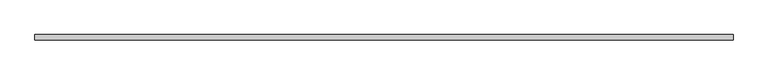
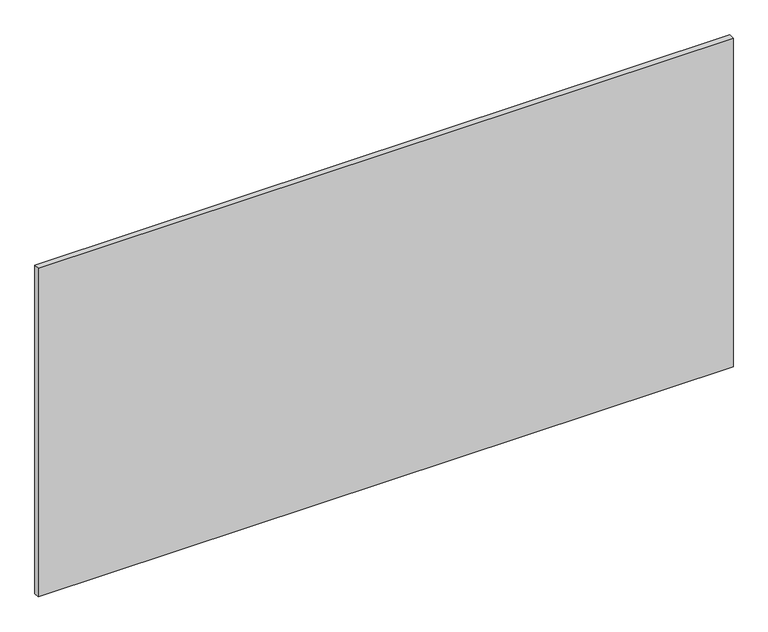
"""IFC4 building model written with IfcOpenShell, lengths in millimetres: proxy geometry, Inner panel:Inner panel:1:Inner panel:1 : Inner panel:Inner panel:300324:300043:Inner panel:1:Inner panel:1 : Inner panel:Inner panel:300324:300043 : Inner panel:Inner panel:1:Inner panel:1 : Inner panel:Inner panel:300324:300043:13 : Inner panel:Inner panel:1:Inner panel:1 : Inner panel:Inner panel:300324:300043:Inner panel:1:Inner panel:1 : Inner panel:Inner panel:300324:300043 : Inner panel:Inner panel:1:Inner panel:1 : Inner panel:Inner panel:300324:300043:300031."""

from ifc_helpers import new_model, si_unit, frame, origin, place, context, project, spatial, polyline, outline, extrude, source, transform, mapped, element, save


def generic_models_36ba1306(model_context):
    return source(origin(), model_context, "Body", "SweptSolid", [
        extrude(outline(polyline([(593738.0867239, -578778.4413841), (596176.4867239, -578778.4413841), (596176.4867239, -578797.4913841), (593738.0867239, -578797.4913841), (593738.0867239, -578778.4413841)])), frame((0.0, 0.0, 2495.55), z_axis=(0.0, 0.0, 1.0), x_axis=(1.0, 0.0, 0.0)), (0.0, 0.0, 1.0), 1219.2),
    ])


if __name__ == "__main__":
    model = new_model("IFC4")
    model_context = context("Model", 3, world=origin())
    ifc_project = project(units=[si_unit("LENGTHUNIT", "METRE", prefix="MILLI")], contexts=[model_context])
    site = spatial("IfcSite", under=ifc_project)
    building = spatial("IfcBuilding", under=site)
    placement = place(None, origin())
    generic_models_shape = generic_models_36ba1306(model_context)
    element("IfcBuildingElementProxy", 1, Name="Inner panel:Inner panel:1:Inner panel:1 : Inner panel:Inner panel:300324:300043:Inner panel:1:Inner panel:1 : Inner panel:Inner panel:300324:300043 : Inner panel:Inner panel:1:Inner panel:1 : Inner panel:Inner panel:300324:300043:13 : Inner panel:Inner panel:1:Inner panel:1 : Inner panel:Inner panel:300324:300043:Inner panel:1:Inner panel:1 : Inner panel:Inner panel:300324:300043 : Inner panel:Inner panel:1:Inner panel:1 : Inner panel:Inner panel:300324:300043:300031", ObjectType="Inner panel:Inner panel:1:Inner panel:1 : Inner panel:Inner panel:300324:300043:Inner panel:1:Inner panel:1 : Inner panel:Inner panel:300324:300043 : Inner panel:Inner panel:1:Inner panel:1 : Inner panel:Inner panel:300324:300043:13 : Inner panel:Inner panel:1:Inner panel:1 : Inner panel:Inner panel:300324:300043:Inner panel:1:Inner panel:1 : Inner panel:Inner panel:300324:300043 : Inner panel:Inner panel:1:Inner panel:1 : Inner panel:Inner panel:300324:300043:300031", at=placement, inside=building, context=model_context, shape_type="MappedRepresentation", body=[
        mapped(generic_models_shape, transform((0.0, 0.0, 0.0), x_axis=(1.0, 0.0, 0.0), y_axis=(0.0, 1.0, 0.0), z_axis=(0.0, 0.0, 1.0))),
    ])
    save(model, "model.ifc")

# Revit data of these elements
# Type "Inner panel:Inner panel:1:Inner panel:1 : Inner panel:Inner panel:300324:300043:Inner panel:1:Inner panel:1 : Inner panel:Inner panel:300324:300043 : Inner panel:Inner panel:1:Inner panel:1 : Inner panel:Inner panel:300324:300043:13 : Inner panel:Inner panel:1:Inner panel:1 : Inner panel:Inner panel:300324:300043:Inner panel:1:Inner panel:1 : Inner panel:Inner panel:300324:300043 : Inner panel:Inner panel:1:Inner panel:1 : Inner panel:Inner panel:300324:300043:300031"
#   NameOverride = "Inner panel:Inner panel:1:Inner panel:1 : Inner panel:Inner panel:300324:300043:Inner panel:1:Inner panel:1 : Inner panel:Inner panel:300324:300043 : Inner panel:Inner panel:1:Inner panel:1 : Inner panel:Inner panel:300324:300043:300031"
#   ObjectTypeOverride = "Inner panel:1:Inner panel:1 : Inner panel:Inner panel:300324:300043 : Inner panel:Inner panel:1:Inner panel:1 : Inner panel:Inner panel:300324:300043"
#   Reference = "Inner panel"
#   Tag = "300031"
# Element 1 (IfcBuildingElementProxy, "Inner panel:Inner panel:1:Inner panel:1 : Inner panel:Inner panel:300324:300043:Inner panel:1:Inner panel:1 : Inner panel:Inner panel:300324:300043 : Inner panel:Inner panel:1:Inner panel:1 : Inner panel:Inner panel:300324:300043:13 : Inner panel:Inner panel:1:Inner panel:1 : Inner panel:Inner panel:300324:300043:Inner panel:1:Inner panel:1 : Inner panel:Inner panel:300324:300043 : Inner panel:Inner panel:1:Inner panel:1 : Inner panel:Inner panel:300324:300043:300031")
#   Materials on its faces: "¾” (CLASS A) FIRE RETARDANT PLYWOOD ...OR… IF 1/4\" GYP. BD UNDER PLYWOOD, FLAME SPREAD TO BE CLASS C -  (FINISH: GRADE B - PREFINISHED STAINED/SEALED) - 1/4\" GAP BTWN PANELS (FASTENERS T.B.D.)"
# Materials
#   "¾” (CLASS A) FIRE RETARDANT PLYWOOD ...OR… IF 1/4\" GYP. BD UNDER PLYWOOD, FLAME SPREAD TO BE CLASS C -  (FINISH: GRADE B - PREFINISHED STAINED/SEALED) - 1/4\" GAP BTWN PANELS (FASTENERS T.B.D.)": class "Wood", colour RGB 149 120 74, transparency 0, Description = "Plywood, sheathing grade", Cost = 0
